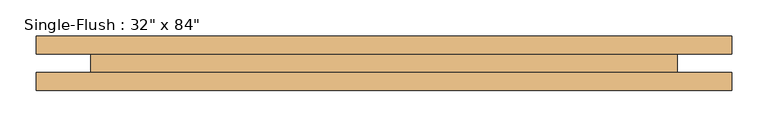
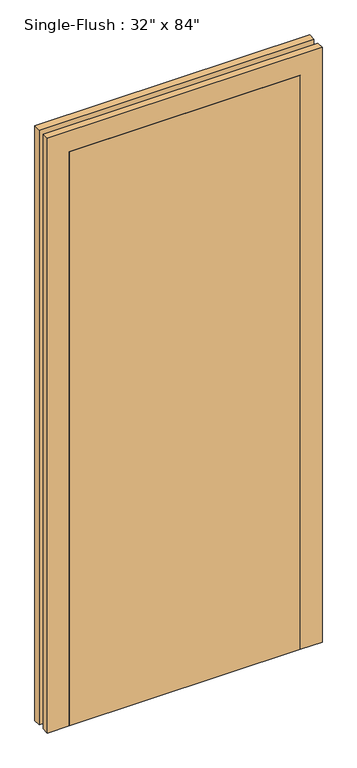
"""IFC4 building model written with IfcOpenShell, lengths in millimetres: door geometry."""

from ifc_helpers import new_model, si_unit, frame, origin, origin_with_axes, place, context, project, spatial, polyline, outline, extrude, source, transform, mapped, element, save


def door_fff709b2(model_context):
    return source(origin(), model_context, "Body", "SweptSolid", [
        extrude(outline(polyline([(2209.8, -482.6), (0.0, -482.6), (0.0, -406.4), (2133.6, -406.4), (2133.6, 406.4), (0.0, 406.4), (0.0, 482.6), (2209.8, 482.6), (2209.8, -482.6)])), frame((0.0, 12.7, 0.0), z_axis=(0.0, 1.0, 0.0), x_axis=(0.0, 0.0, 1.0)), (0.0, 0.0, 1.0), 25.4),
        extrude(outline(polyline([(2209.8, 482.6), (2209.8, -482.6), (0.0, -482.6), (0.0, -406.4), (2133.6, -406.4), (2133.6, 406.4), (0.0, 406.4), (0.0, 482.6), (2209.8, 482.6)])), frame((0.0, -38.1, 0.0), z_axis=(0.0, 1.0, 0.0), x_axis=(0.0, 0.0, 1.0)), (0.0, 0.0, 1.0), 25.4),
        extrude(outline(polyline([(406.4, -38.1), (-406.4, -38.1), (-406.4, 12.7), (406.4, 12.7), (406.4, -38.1)])), origin_with_axes(), (0.0, 0.0, 1.0), 2133.6),
    ])


if __name__ == "__main__":
    model = new_model("IFC4")
    model_context = context("Model", 3, world=origin())
    ifc_project = project(units=[si_unit("LENGTHUNIT", "METRE", prefix="MILLI")], contexts=[model_context])
    site = spatial("IfcSite", under=ifc_project)
    building = spatial("IfcBuilding", under=site)
    placement = place(None, origin())
    door_shape = door_fff709b2(model_context)
    element("IfcDoor", 1, ObjectType="Single-Flush : 32\" x 84\"", at=placement, inside=building, context=model_context, shape_type="MappedRepresentation", body=[
        mapped(door_shape, transform((0.0, 0.0, 0.0), x_axis=(1.0, 0.0, 0.0), y_axis=(0.0, 1.0, 0.0), z_axis=(0.0, 0.0, 1.0))),
    ])
    save(model, "model.ifc")

# Revit data of these elements
# Type "Single-Flush : 32\" x 84\""
#   Type Mark = "10"
#   Construction Type Id = "MDOOR"
#   Assembly Code = "C1020"
#   Analytic Construction = "Metal"
#   Thickness = 0' - 2"
#   Heat Transfer Coefficient (U) = 3.7021 W/(m²·K)
#   Height = 7' - 0"
#   Trim Projection Ext = 0' - 1"
#   Trim Projection Int = 0' - 1"
#   Trim Width = 0' - 3"
#   Width = 2' - 8"
#   Door Material = Door - Panel
#   Frame Material = Door - Frame
#   Visual Light Transmittance = 0
#   Solar Heat Gain Coefficient = 0
#   Function = (empty or 0)
#   Wall Closure = (empty or 0)
# Element 1 (IfcDoor, "Single-Flush : 32\" x 84\"")
#   Materials on its faces: "Door - Frame", "Door - Panel"
# Materials
#   "Door - Panel": class "Wood", colour RGB 210 159 95, transparency 0
#   "Door - Frame": class "Miscellaneous", colour RGB 118 70 51, transparency 0
